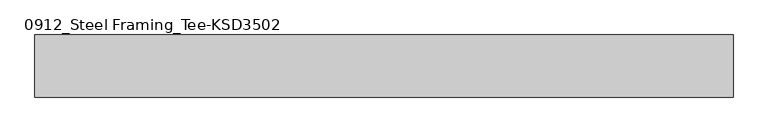
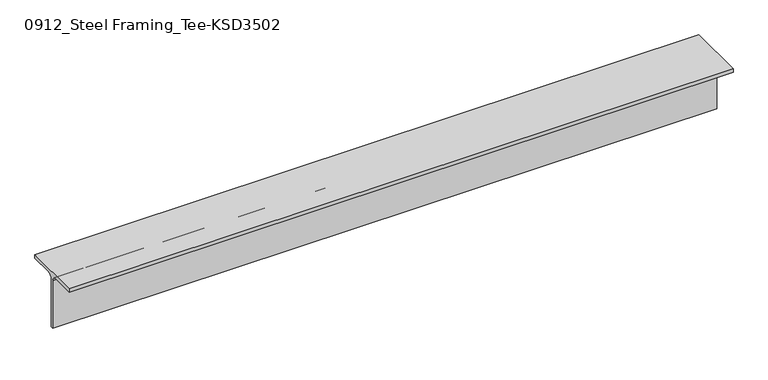
"""IFC4 building model written with IfcOpenShell, lengths in millimetres: member geometry, 0912_Steel Framing_Tee-KSD3502 : H_SB_ASB_CT-150x150x6.5x9."""

from ifc_helpers import new_model, si_unit, point, frame, frame_2d, origin, place, context, project, spatial, polyline, circle_curve, trimmed, segment, composite_curve, outline, extrude, source, transform, mapped, element, save


def member_0912_steel_framing_tee_ksd3502_44a8cdcd(model_context):
    return source(origin(), model_context, "Body", "SweptSolid", [
        extrude(outline(composite_curve([segment(polyline([(75.0, 75.0), (75.0, 66.0), (16.25, 66.0)]), True, "CONTINUOUS"), segment(trimmed(circle_curve(frame_2d((16.25, 53.0)), 13.0), [point((16.25, 66.0))], [point((3.25, 53.0))], True, "CARTESIAN"), True, "CONTINUOUS"), segment(polyline([(3.25, 53.0), (3.25, -75.0), (-3.25, -75.0), (-3.25, 53.0)]), True, "CONTINUOUS"), segment(trimmed(circle_curve(frame_2d((-16.25, 53.0)), 13.0), [point((-3.25, 53.0))], [point((-16.25, 66.0))], True, "CARTESIAN"), True, "CONTINUOUS"), segment(polyline([(-16.25, 66.0), (-75.0, 66.0), (-75.0, 75.0), (75.0, 75.0)]), True, "CONTINUOUS")], self_intersect=False)), frame((-842.3, 0.0, 0.0), z_axis=(1.0, 0.0, 0.0), x_axis=(0.0, 1.0, 0.0)), (0.0, 0.0, 1.0), 1684.6),
    ])


if __name__ == "__main__":
    model = new_model("IFC4")
    model_context = context("Model", 3, world=origin())
    ifc_project = project(units=[si_unit("LENGTHUNIT", "METRE", prefix="MILLI")], contexts=[model_context])
    site = spatial("IfcSite", under=ifc_project)
    building = spatial("IfcBuilding", under=site)
    placement = place(None, origin())
    member_0912_steel_framing_tee_ksd3502_shape = member_0912_steel_framing_tee_ksd3502_44a8cdcd(model_context)
    element("IfcMember", 1, ObjectType="0912_Steel Framing_Tee-KSD3502 : H_SB_ASB_CT-150x150x6.5x9", at=placement, inside=building, context=model_context, shape_type="MappedRepresentation", body=[
        mapped(member_0912_steel_framing_tee_ksd3502_shape, transform((0.0, 0.0, 0.0), x_axis=(1.0, 0.0, 0.0), y_axis=(0.0, 1.0, 0.0), z_axis=(0.0, 0.0, 1.0))),
    ])
    save(model, "model.ifc")

# Revit data of these elements
# Type "0912_Steel Framing_Tee-KSD3502 : H_SB_ASB_CT-150x150x6.5x9"
#   H_WM Code_1 = "S01AA003-00001 | Main Steel Structure Fabrication Work | Shelter/Building | Light Steel - Standard (30KG/M>Weight) | Material: (   )"
#   H_WM Code_2 = "S03AA029-00001 | Main Steel Structure Erection Work | Shelter/Building | Light Steel (30KG/M>Weight) | Material: (   )"
#   H_WM Code_3 = "S01AA010-00001 | Main Steel Structure Fabrication Work | Shelter/Building | Steel Painting/Coating | for Non-Fireproofed Steel Surface, Surface Preparation, Primer, Second & Final Coat | Material: (   )"
#   H_Q'ty Cal Type Tag = "SB-Q2"
#   Width = 15.0 cm
#   Web Thickness = 0.65 cm
#   Web Fillet = 1.3 cm
#   Section Area = 23.39 cm²
#   Perimeter = 0.60 m²/m
#   Nominal Weight = 18.40 kgf/m
#   Height = 15.0 cm
#   Flange Thickness = 0.9 cm
#   Centroid Vertical = 7.5 cm
#   Centroid Horizontal = 7.5 cm
#   Length [instance default] = 1.5000 m
#   Structural Material [instance default] = Steel, 45-345
#   Warping Constant = (empty or 0)
#   Torsional Moment of Inertia = 0
#   Section Name Key = ""
#   Plastic Modulus weak axis = 0
#   Plastic Modulus strong axis = 0
#   Moment of Inertia weak axis = 0
#   Moment of Inertia strong axis = 0
#   Elastic Modulus weak axis = 0
#   Elastic Modulus strong axis = 0
#   Bolt Spacing = 0
#   Assembly Code = ""
# Element 1 (IfcMember, "0912_Steel Framing_Tee-KSD3502 : H_SB_ASB_CT-150x150x6.5x9")
#   Structural Material = none
# Materials
#   "Steel, 45-345": class "Metal", colour RGB 189 187 185, transparency 0, Description = "Steel 345 MPa", Cost = 0
